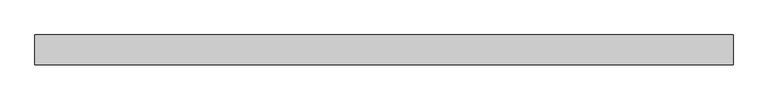
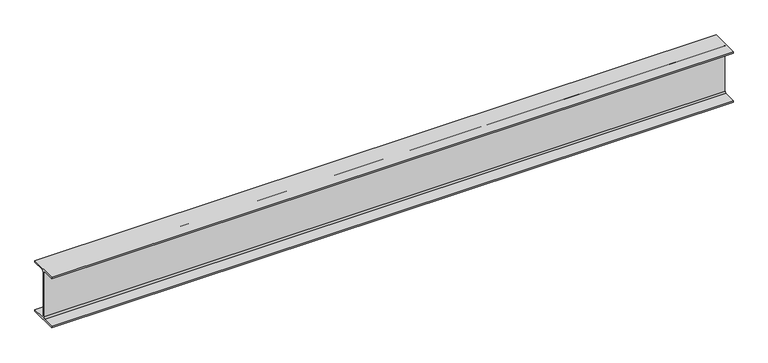
"""IFC4 building model written with IfcOpenShell, lengths in millimetres: beam geometry, Old_Steel Beam_H-KSD3502 : H_SB_ASB_H-250×125x6x9."""

from ifc_helpers import new_model, si_unit, point, frame, frame_2d, origin, place, context, project, spatial, polyline, circle_curve, trimmed, segment, composite_curve, outline, extrude, source, transform, mapped, element, save


def beam_4107c911(model_context):
    return source(origin(), model_context, "Body", "SweptSolid", [
        extrude(outline(composite_curve([segment(polyline([(82.5, -141.5), (82.5, -151.7), (-82.5, -151.7), (-82.5, -141.5), (-11.9, -141.5)]), True, "CONTINUOUS"), segment(trimmed(circle_curve(frame_2d((-11.9, -132.6)), 8.9), [point((-11.9, -141.5))], [point((-3.0, -132.6))], True, "CARTESIAN"), True, "CONTINUOUS"), segment(polyline([(-3.0, -132.6), (-3.0, 132.6)]), True, "CONTINUOUS"), segment(trimmed(circle_curve(frame_2d((-11.9, 132.6)), 8.9), [point((-3.0, 132.6))], [point((-11.9, 141.5))], True, "CARTESIAN"), True, "CONTINUOUS"), segment(polyline([(-11.9, 141.5), (-82.5, 141.5), (-82.5, 151.7), (82.5, 151.7), (82.5, 141.5), (11.9, 141.5)]), True, "CONTINUOUS"), segment(trimmed(circle_curve(frame_2d((11.9, 132.6)), 8.9), [point((11.9, 141.5))], [point((3.0, 132.6))], True, "CARTESIAN"), True, "CONTINUOUS"), segment(polyline([(3.0, 132.6), (3.0, -132.6)]), True, "CONTINUOUS"), segment(trimmed(circle_curve(frame_2d((11.9, -132.6)), 8.9), [point((3.0, -132.6))], [point((11.9, -141.5))], True, "CARTESIAN"), True, "CONTINUOUS"), segment(polyline([(11.9, -141.5), (82.5, -141.5)]), True, "CONTINUOUS")], self_intersect=False)), frame((-1830.0827532, 0.0, 0.0), z_axis=(1.0, 0.0, 0.0), x_axis=(0.0, 1.0, 0.0)), (0.0, 0.0, 1.0), 3859.8827532),
    ])


if __name__ == "__main__":
    model = new_model("IFC4")
    model_context = context("Model", 3, world=origin())
    ifc_project = project(units=[si_unit("LENGTHUNIT", "METRE", prefix="MILLI")], contexts=[model_context])
    site = spatial("IfcSite", under=ifc_project)
    building = spatial("IfcBuilding", under=site)
    placement = place(None, origin())
    beam_shape = beam_4107c911(model_context)
    element("IfcBeam", 1, ObjectType="Old_Steel Beam_H-KSD3502 : H_SB_ASB_H-250×125x6x9", at=placement, inside=building, context=model_context, shape_type="MappedRepresentation", body=[
        mapped(beam_shape, transform((0.0, 0.0, 0.0), x_axis=(1.0, 0.0, 0.0), y_axis=(0.0, 1.0, 0.0), z_axis=(0.0, 0.0, 1.0))),
    ])
    save(model, "model.ifc")

# Revit data of these elements
# Type "Old_Steel Beam_H-KSD3502 : H_SB_ASB_H-250×125x6x9"
#   Width = 12.5 cm
#   Web Thickness = 0.6 cm
#   Web Fillet = 1.2 cm
#   Warping Constant = 42539.8 cm⁶
#   Torsional Moment of Inertia = 7.8102 cm⁴
#   Torsional Modulus = 1.0 cm³
#   Section Area = 37.66 cm²
#   Plastic Modulus weak axis = 73.1 cm³
#   Plastic Modulus strong axis = 366.0 cm³
#   Perimeter = 0.97 m²/m
#   Nominal Weight = 29.60 kgf/m
#   Moment of Inertia weak axis = 294.00 cm⁴
#   Moment of Inertia strong axis = 4050.00 cm⁴
#   Height = 25.0 cm
#   Flange Thickness = 0.9 cm
#   Elastic Modulus weak axis = 47.0 cm³
#   Elastic Modulus strong axis = 324.0 cm³
#   Centroid Vertical = 12.5 cm
#   Centroid Horizontal = 6.25 cm
#   Length [instance default] = 1.5240 m
#   Structural Material [instance default] = Steel, 45-345
#   Assembly Code = ""
# Element 1 (IfcBeam, "Old_Steel Beam_H-KSD3502 : H_SB_ASB_H-250×125x6x9")
#   Structural Material = none
# Materials
#   "Steel, 45-345": class "Metal", colour RGB 189 187 185, transparency 0, Description = "Steel 345 MPa", Cost = 0
